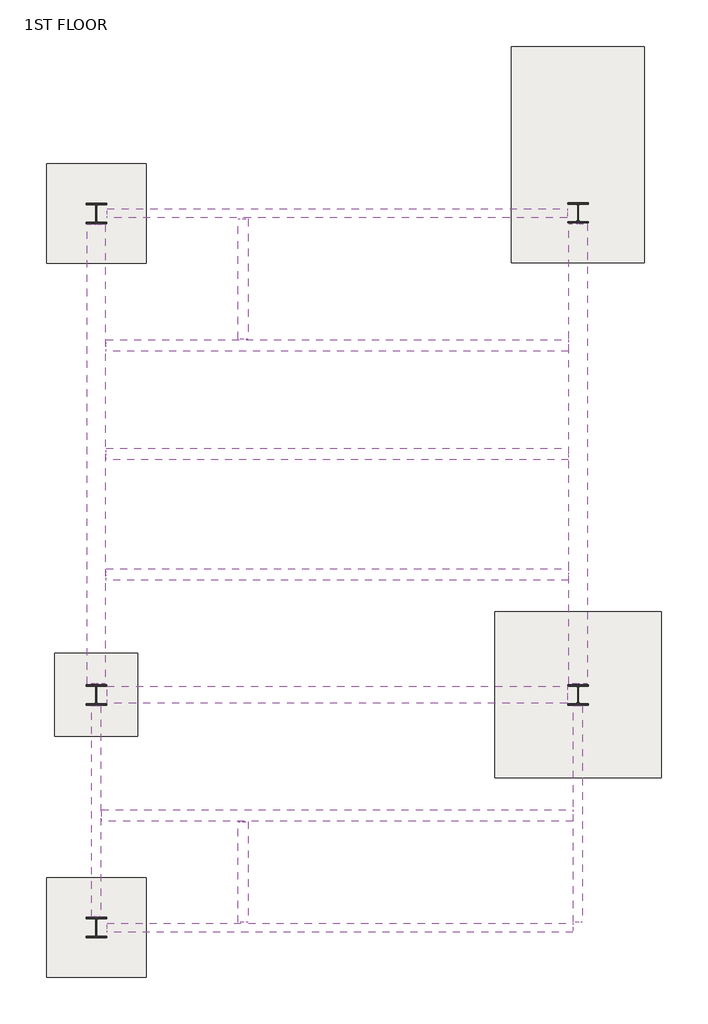
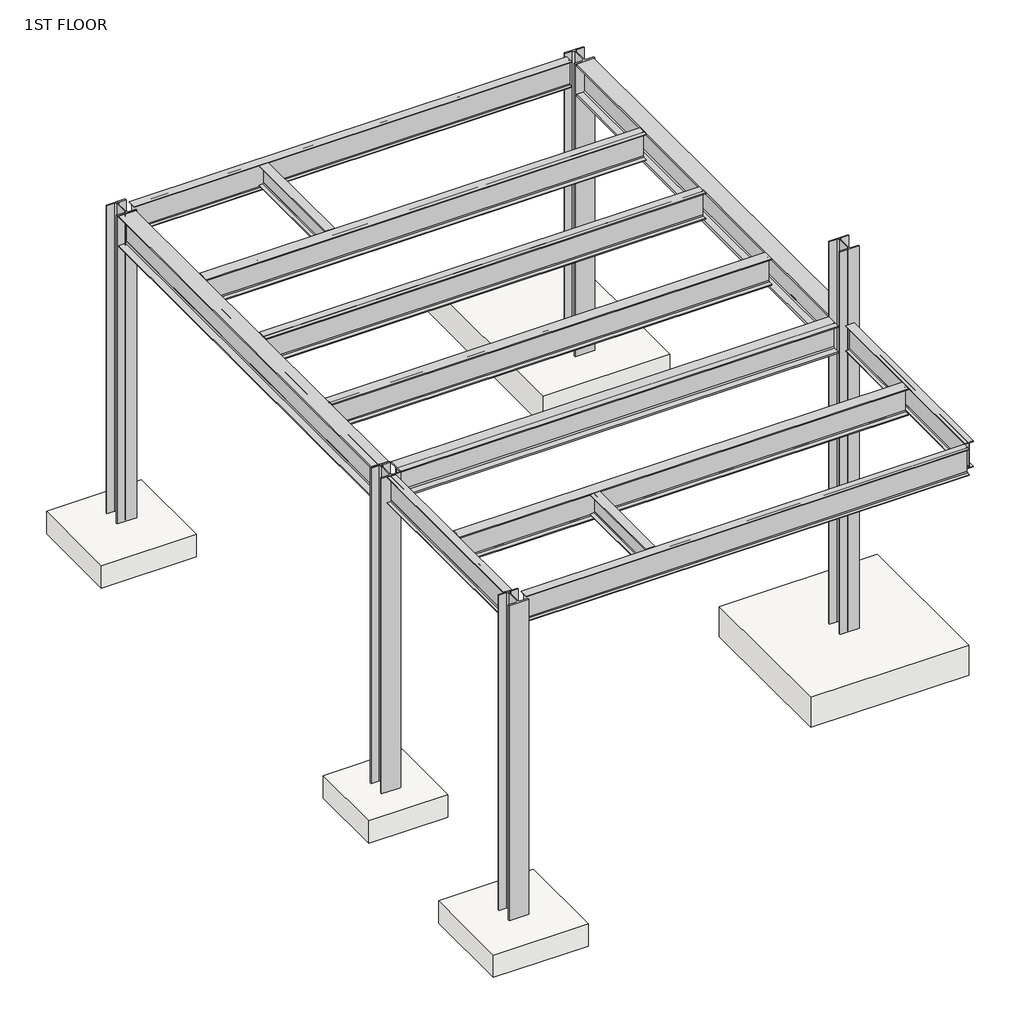
# One storey: 13 beams, 5 columns, 5 slabs.
"""IFC4 building model written with IfcOpenShell, lengths in millimetres."""

import ifcopenshell
import ifcopenshell.guid

model = None  # the IFC model being written
_history = None  # IfcOwnerHistory: only IFC2X3 demands one
_inside = {}  # id of a spatial element -> (the spatial element, [elements in it])
_under = {}  # id of a project, library or spatial element -> (it, [spatial elements below it])
_declared = {}  # id of a project -> (the project, [libraries it declares])
_typed = {}  # id of a type object -> (the type object, [elements of that type])
_made_of = {}  # id of a material, layer set ... -> (it, [elements and type objects made of it])


def new_model(schema):
    """Start an empty IFC model of exactly this schema.

    Asked for "IFC4X3", IfcOpenShell would pick the latest addendum, in which some entities
    have other attributes; the version numbers below select the first issue.
    IFC2X3 requires an IfcOwnerHistory on every rooted entity: one is made here for all.
    """
    global model, _history
    if schema == "IFC4X3":
        model = ifcopenshell.file(schema_version=(4, 3, 0, 0))
    else:
        model = ifcopenshell.file(schema=schema)
    _inside.clear()
    _under.clear()
    _declared.clear()
    _typed.clear()
    _made_of.clear()
    _history = None
    if model.schema == "IFC2X3":
        org = make("IfcOrganization", Name="unknown")
        user = make(
            "IfcPersonAndOrganization",
            ThePerson=make("IfcPerson", FamilyName="unknown"),
            TheOrganization=org,
        )
        app = make(
            "IfcApplication",
            ApplicationDeveloper=org,
            Version="unknown",
            ApplicationFullName="unknown",
            ApplicationIdentifier="unknown",
        )
        _history = make(
            "IfcOwnerHistory",
            OwningUser=user,
            OwningApplication=app,
            ChangeAction="ADDED",
            CreationDate=0,
        )
    return model


def make(cls, **values):
    """One entity of the class cls with the attributes given. An attribute that is None is left unset."""
    return model.create_entity(
        cls, **{name: value for name, value in values.items() if value is not None}
    )


def rooted(cls, **values):
    """An entity with a GlobalId (a new one), such as an element, a storey or a relation."""
    return make(cls, GlobalId=ifcopenshell.guid.new(), OwnerHistory=_history, **values)


def si_unit(unit_type, name, prefix=None):
    """IfcSIUnit, for example si_unit("LENGTHUNIT", "METRE", prefix="MILLI")."""
    return make("IfcSIUnit", UnitType=unit_type, Prefix=prefix, Name=name)


def assignment(units):
    """IfcUnitAssignment: the units of a project."""
    return None if units is None else make("IfcUnitAssignment", Units=units)


def point(xyz):
    """IfcCartesianPoint."""
    return None if xyz is None else make("IfcCartesianPoint", Coordinates=xyz)


def direction(xyz):
    """IfcDirection."""
    return None if xyz is None else make("IfcDirection", DirectionRatios=xyz)


def frame(location, z_axis=None, x_axis=None):
    """IfcAxis2Placement3D, a coordinate frame: its origin and axes. An axis left out is left unset."""
    return make(
        "IfcAxis2Placement3D",
        Location=point(location),
        Axis=direction(z_axis),
        RefDirection=direction(x_axis),
    )


def frame_2d(location, x_axis=None):
    """IfcAxis2Placement2D, a coordinate frame in the plane: its origin and x axis."""
    return make(
        "IfcAxis2Placement2D", Location=point(location), RefDirection=direction(x_axis)
    )


def origin():
    """The frame at (0, 0, 0) with its axes left unset."""
    return frame((0.0, 0.0, 0.0))


def origin_with_axes():
    """The frame at (0, 0, 0) with the z axis (0, 0, 1) and the x axis (1, 0, 0) written out."""
    return frame((0.0, 0.0, 0.0), z_axis=(0.0, 0.0, 1.0), x_axis=(1.0, 0.0, 0.0))


def place(relative_to, where):
    """IfcLocalPlacement: puts the frame where relative to a parent placement (None: the world)."""
    return make(
        "IfcLocalPlacement", PlacementRelTo=relative_to, RelativePlacement=where
    )


def context(
    kind, dimensions, precision=None, world=None, true_north=None, identifier=None
):
    """IfcGeometricRepresentationContext, for example the 3D "Model" context."""
    return make(
        "IfcGeometricRepresentationContext",
        ContextIdentifier=identifier,
        ContextType=kind,
        CoordinateSpaceDimension=dimensions,
        Precision=precision,
        WorldCoordinateSystem=world,
        TrueNorth=true_north,
    )


def project(units=None, contexts=None):
    """IfcProject with its units and contexts."""
    return rooted(
        "IfcProject",
        Name="project",
        RepresentationContexts=contexts,
        UnitsInContext=assignment(units),
    )


def spatial(cls, under=None, at=None, **own):
    """A site, building, storey or space (cls), placed at a placement, below another one or the project."""
    s = rooted(cls, ObjectPlacement=at, **own)
    if under is not None:
        _under.setdefault(under.id(), (under, []))[1].append(s)
    return s


def polyline(points):
    """IfcPolyline through the points."""
    return make("IfcPolyline", Points=[point(p) for p in points])


def circle_curve(where, radius):
    """IfcCircle in the frame where."""
    return make("IfcCircle", Position=where, Radius=radius)


def trimmed(basis, trim1, trim2, sense, master):
    """IfcTrimmedCurve: the piece of a basis curve between two trims."""
    return make(
        "IfcTrimmedCurve",
        BasisCurve=basis,
        Trim1=trim1,
        Trim2=trim2,
        SenseAgreement=sense,
        MasterRepresentation=master,
    )


def segment(curve, same_sense, transition):
    """IfcCompositeCurveSegment."""
    return make(
        "IfcCompositeCurveSegment",
        Transition=transition,
        SameSense=same_sense,
        ParentCurve=curve,
    )


def composite_curve(segments, self_intersect=None):
    """IfcCompositeCurve: segments joined end to end."""
    return make("IfcCompositeCurve", Segments=segments, SelfIntersect=self_intersect)


def outline(outer, holes=None, kind="AREA"):
    """IfcArbitraryClosedProfileDef: a profile drawn as a closed curve; with holes, ...WithVoids."""
    if holes is None:
        return make("IfcArbitraryClosedProfileDef", ProfileType=kind, OuterCurve=outer)
    return make(
        "IfcArbitraryProfileDefWithVoids",
        ProfileType=kind,
        OuterCurve=outer,
        InnerCurves=holes,
    )


def extrude(swept, where, along, depth):
    """IfcExtrudedAreaSolid: the profile swept, set in the frame where, extruded along a direction by depth."""
    return make(
        "IfcExtrudedAreaSolid",
        SweptArea=swept,
        Position=where,
        ExtrudedDirection=direction(along),
        Depth=depth,
    )


def shape(context_of_items, identifier, shape_type, items):
    """IfcShapeRepresentation: the items that make up one representation, for example the "Body"."""
    return make(
        "IfcShapeRepresentation",
        ContextOfItems=context_of_items,
        RepresentationIdentifier=identifier,
        RepresentationType=shape_type,
        Items=items,
    )


def source(mapping_origin, context_of_items, identifier, shape_type, items):
    """IfcRepresentationMap: a shape defined once, which mapped items show again and again."""
    return make(
        "IfcRepresentationMap",
        MappingOrigin=mapping_origin,
        MappedRepresentation=shape(context_of_items, identifier, shape_type, items),
    )


def transform(
    local_origin,
    x_axis=None,
    y_axis=None,
    z_axis=None,
    scale=None,
    scale2=None,
    scale3=None,
    uniform=True,
):
    """IfcCartesianTransformationOperator3D, or its non-uniform kind. x_axis, y_axis, z_axis: its Axis1, 2, 3."""
    if uniform:
        return make(
            "IfcCartesianTransformationOperator3D",
            Axis1=direction(x_axis),
            Axis2=direction(y_axis),
            LocalOrigin=point(local_origin),
            Scale=scale,
            Axis3=direction(z_axis),
        )
    return make(
        "IfcCartesianTransformationOperator3DnonUniform",
        Axis1=direction(x_axis),
        Axis2=direction(y_axis),
        LocalOrigin=point(local_origin),
        Scale=scale,
        Axis3=direction(z_axis),
        Scale2=scale2,
        Scale3=scale3,
    )


def mapped(mapping_source, mapping_target):
    """IfcMappedItem: shows the shape of a source again, moved by a transform."""
    return make(
        "IfcMappedItem", MappingSource=mapping_source, MappingTarget=mapping_target
    )


def made_of(thing, what):
    """Note that an element or type object is made of a material, layer set ...; save() writes the relation."""
    if what is not None:
        _made_of.setdefault(what.id(), (what, []))[1].append(thing)
    return thing


def element(
    cls,
    number,
    at=None,
    inside=None,
    cuts=None,
    type_object=None,
    material=None,
    context=None,
    identifier="Body",
    shape_type=None,
    held_by="IfcProductDefinitionShape",
    body=None,
    shapes=None,
    **own,
):
    """One element of the class cls, such as IfcWall. Its Tag is "e" and its number.

    at: its placement. inside: the storey or other place that contains it. cuts: it is an
    opening in that element (IfcRelVoidsElement). A single representation is given by context,
    identifier, shape_type and body (its items); several are given by shapes. held_by: the class
    of the entity that holds the representations. save() writes the other relations.
    """
    e = rooted(cls, Tag="e%d" % number, ObjectPlacement=at, **own)
    if body is not None:
        shapes = [shape(context, identifier, shape_type, body)]
    if shapes is not None:
        e.Representation = make(held_by, Representations=shapes)
    if inside is not None:
        _inside.setdefault(inside.id(), (inside, []))[1].append(e)
    if cuts is not None:
        rooted(
            "IfcRelVoidsElement", RelatingBuildingElement=cuts, RelatedOpeningElement=e
        )
    if type_object is not None:
        _typed.setdefault(type_object.id(), (type_object, []))[1].append(e)
    return made_of(e, material)


def aggregate(whole, parts):
    """IfcRelAggregates: a whole, such as a stair, and the parts it consists of."""
    return rooted("IfcRelAggregates", RelatingObject=whole, RelatedObjects=parts)


def save(model, path):
    """Write the relations noted so far, then the file.

    IfcRelAggregates (storeys below a building ...), IfcRelContainedInSpatialStructure (elements
    in a storey), IfcRelDefinesByType, IfcRelAssociatesMaterial and IfcRelDeclares: one each for
    every whole, place, type object, material and project.
    """
    for whole, parts in _under.values():
        aggregate(whole, parts)
    for where, things in _inside.values():
        rooted(
            "IfcRelContainedInSpatialStructure",
            RelatedElements=things,
            RelatingStructure=where,
        )
    for kind, things in _typed.values():
        rooted("IfcRelDefinesByType", RelatedObjects=things, RelatingType=kind)
    for what, things in _made_of.values():
        rooted("IfcRelAssociatesMaterial", RelatedObjects=things, RelatingMaterial=what)
    for by, libraries in _declared.values():
        rooted("IfcRelDeclares", RelatingContext=by, RelatedDefinitions=libraries)
    model.write(path)


def w_wide_flange_w16x50_2f8f61bc(model_context):
    return source(origin(), model_context, "Body", "SweptSolid", [
        extrude(outline(composite_curve([segment(polyline([(89.789, -191.008), (89.789, -207.01), (-89.789, -207.01), (-89.789, -191.008), (-22.1615, -191.008)]), True, "CONTINUOUS"), segment(trimmed(circle_curve(frame_2d((-22.1615, -173.6725)), 17.3355), [point((-22.1615, -191.008))], [point((-4.826, -173.6725))], True, "CARTESIAN"), True, "CONTINUOUS"), segment(polyline([(-4.826, -173.6725), (-4.826, 173.6725)]), True, "CONTINUOUS"), segment(trimmed(circle_curve(frame_2d((-22.1615, 173.6725)), 17.3355), [point((-4.826, 173.6725))], [point((-22.1615, 191.008))], True, "CARTESIAN"), True, "CONTINUOUS"), segment(polyline([(-22.1615, 191.008), (-89.789, 191.008), (-89.789, 207.01), (89.789, 207.01), (89.789, 191.008), (22.1615, 191.008)]), True, "CONTINUOUS"), segment(trimmed(circle_curve(frame_2d((22.1615, 173.6725)), 17.3355), [point((22.1615, 191.008))], [point((4.826, 173.6725))], True, "CARTESIAN"), True, "CONTINUOUS"), segment(polyline([(4.826, 173.6725), (4.826, -173.6725)]), True, "CONTINUOUS"), segment(trimmed(circle_curve(frame_2d((22.1615, -173.6725)), 17.3355), [point((4.826, -173.6725))], [point((22.1615, -191.008))], True, "CARTESIAN"), True, "CONTINUOUS"), segment(polyline([(22.1615, -191.008), (89.789, -191.008)]), True, "CONTINUOUS")], self_intersect=False)), frame((-1094.5030758, 0.0, 0.0), z_axis=(1.0, 0.0, 0.0), x_axis=(0.0, 1.0, 0.0)), (0.0, 0.0, 1.0), 2211.8661516),
    ])


def w_wide_flange_w16x50_f430b839(model_context):
    return source(origin(), model_context, "Body", "SweptSolid", [
        extrude(outline(composite_curve([segment(polyline([(-89.789, -191.008), (-22.1615, -191.008)]), True, "CONTINUOUS"), segment(trimmed(circle_curve(frame_2d((-22.1615, -173.6725)), 17.3355), [point((-22.1615, -191.008))], [point((-4.826, -173.6725))], True, "CARTESIAN"), True, "CONTINUOUS"), segment(polyline([(-4.826, -173.6725), (-4.826, 173.6725)]), True, "CONTINUOUS"), segment(trimmed(circle_curve(frame_2d((-22.1615, 173.6725)), 17.3355), [point((-4.826, 173.6725))], [point((-22.1615, 191.008))], True, "CARTESIAN"), True, "CONTINUOUS"), segment(polyline([(-22.1615, 191.008), (-89.789, 191.008), (-89.789, 207.01), (89.789, 207.01), (89.789, 191.008), (22.1615, 191.008)]), True, "CONTINUOUS"), segment(trimmed(circle_curve(frame_2d((22.1615, 173.6725)), 17.3355), [point((22.1615, 191.008))], [point((4.826, 173.6725))], True, "CARTESIAN"), True, "CONTINUOUS"), segment(polyline([(4.826, 173.6725), (4.826, -173.6725)]), True, "CONTINUOUS"), segment(trimmed(circle_curve(frame_2d((22.1615, -173.6725)), 17.3355), [point((4.826, -173.6725))], [point((22.1615, -191.008))], True, "CARTESIAN"), True, "CONTINUOUS"), segment(polyline([(22.1615, -191.008), (89.789, -191.008), (89.789, -207.01), (-89.789, -207.01), (-89.789, -191.008)]), True, "CONTINUOUS")], self_intersect=False)), frame((-912.045346, 0.0, 0.0), z_axis=(1.0, 0.0, 0.0), x_axis=(0.0, 1.0, 0.0)), (0.0, 0.0, 1.0), 1846.950692),
    ])


def w_wide_flange_w21x111_51b1a384(model_context):
    return source(origin(), model_context, "Body", "SweptSolid", [
        extrude(outline(composite_curve([segment(polyline([(156.21, -250.825), (156.21, -273.05), (-156.21, -273.05), (-156.21, -250.825), (-29.21, -250.825)]), True, "CONTINUOUS"), segment(trimmed(circle_curve(frame_2d((-29.21, -228.6)), 22.225), [point((-29.21, -250.825))], [point((-6.985, -228.6))], True, "CARTESIAN"), True, "CONTINUOUS"), segment(polyline([(-6.985, -228.6), (-6.985, 228.6)]), True, "CONTINUOUS"), segment(trimmed(circle_curve(frame_2d((-29.21, 228.6)), 22.225), [point((-6.985, 228.6))], [point((-29.21, 250.825))], True, "CARTESIAN"), True, "CONTINUOUS"), segment(polyline([(-29.21, 250.825), (-156.21, 250.825), (-156.21, 273.05), (156.21, 273.05), (156.21, 250.825), (29.21, 250.825)]), True, "CONTINUOUS"), segment(trimmed(circle_curve(frame_2d((29.21, 228.6)), 22.225), [point((29.21, 250.825))], [point((6.985, 228.6))], True, "CARTESIAN"), True, "CONTINUOUS"), segment(polyline([(6.985, 228.6), (6.985, -228.6)]), True, "CONTINUOUS"), segment(trimmed(circle_curve(frame_2d((29.21, -228.6)), 22.225), [point((6.985, -228.6))], [point((29.21, -250.825))], True, "CARTESIAN"), True, "CONTINUOUS"), segment(polyline([(29.21, -250.825), (156.21, -250.825)]), True, "CONTINUOUS")], self_intersect=False)), frame((-4220.21, 0.0, 0.0), z_axis=(1.0, 0.0, 0.0), x_axis=(0.0, 1.0, 0.0)), (0.0, 0.0, 1.0), 8440.42),
    ])


def w_wide_flange_w21x44_feb090a0(model_context):
    return source(origin(), model_context, "Body", "SweptSolid", [
        extrude(outline(composite_curve([segment(polyline([(82.55, -251.46), (82.55, -262.89), (-82.55, -262.89), (-82.55, -251.46), (-21.59, -251.46)]), True, "CONTINUOUS"), segment(trimmed(circle_curve(frame_2d((-21.59, -234.315)), 17.145), [point((-21.59, -251.46))], [point((-4.445, -234.315))], True, "CARTESIAN"), True, "CONTINUOUS"), segment(polyline([(-4.445, -234.315), (-4.445, 234.315)]), True, "CONTINUOUS"), segment(trimmed(circle_curve(frame_2d((-21.59, 234.315)), 17.145), [point((-4.445, 234.315))], [point((-21.59, 251.46))], True, "CARTESIAN"), True, "CONTINUOUS"), segment(polyline([(-21.59, 251.46), (-82.55, 251.46), (-82.55, 262.89), (82.55, 262.89), (82.55, 251.46), (21.59, 251.46)]), True, "CONTINUOUS"), segment(trimmed(circle_curve(frame_2d((21.59, 234.315)), 17.145), [point((21.59, 251.46))], [point((4.445, 234.315))], True, "CARTESIAN"), True, "CONTINUOUS"), segment(polyline([(4.445, 234.315), (4.445, -234.315)]), True, "CONTINUOUS"), segment(trimmed(circle_curve(frame_2d((21.59, -234.315)), 17.145), [point((4.445, -234.315))], [point((21.59, -251.46))], True, "CARTESIAN"), True, "CONTINUOUS"), segment(polyline([(21.59, -251.46), (82.55, -251.46)]), True, "CONTINUOUS")], self_intersect=False)), frame((-4220.21, 0.0, 0.0), z_axis=(1.0, 0.0, 0.0), x_axis=(0.0, 1.0, 0.0)), (0.0, 0.0, 1.0), 8440.42),
    ])


def w_wide_flange_w21x44_b9bda158(model_context):
    return source(origin(), model_context, "Body", "SweptSolid", [
        extrude(outline(composite_curve([segment(polyline([(82.55, -251.46), (82.55, -262.89), (-82.55, -262.89), (-82.55, -251.46), (-21.59, -251.46)]), True, "CONTINUOUS"), segment(trimmed(circle_curve(frame_2d((-21.59, -234.315)), 17.145), [point((-21.59, -251.46))], [point((-4.445, -234.315))], True, "CARTESIAN"), True, "CONTINUOUS"), segment(polyline([(-4.445, -234.315), (-4.445, 234.315)]), True, "CONTINUOUS"), segment(trimmed(circle_curve(frame_2d((-21.59, 234.315)), 17.145), [point((-4.445, 234.315))], [point((-21.59, 251.46))], True, "CARTESIAN"), True, "CONTINUOUS"), segment(polyline([(-21.59, 251.46), (-82.55, 251.46), (-82.55, 262.89), (82.55, 262.89), (82.55, 251.46), (21.59, 251.46)]), True, "CONTINUOUS"), segment(trimmed(circle_curve(frame_2d((21.59, 234.315)), 17.145), [point((21.59, 251.46))], [point((4.445, 234.315))], True, "CARTESIAN"), True, "CONTINUOUS"), segment(polyline([(4.445, 234.315), (4.445, -234.315)]), True, "CONTINUOUS"), segment(trimmed(circle_curve(frame_2d((21.59, -234.315)), 17.145), [point((4.445, -234.315))], [point((21.59, -251.46))], True, "CARTESIAN"), True, "CONTINUOUS"), segment(polyline([(21.59, -251.46), (82.55, -251.46)]), True, "CONTINUOUS")], self_intersect=False)), frame((-1935.665346, 0.0, 0.0), z_axis=(1.0, 0.0, 0.0), x_axis=(0.0, 1.0, 0.0)), (0.0, 0.0, 1.0), 3868.155692),
    ])


def w_wide_flange_w21x44_85607f17(model_context):
    return source(origin(), model_context, "Body", "SweptSolid", [
        extrude(outline(composite_curve([segment(polyline([(82.55, -251.46), (82.55, -262.89), (-82.55, -262.89), (-82.55, -251.46), (-21.59, -251.46)]), True, "CONTINUOUS"), segment(trimmed(circle_curve(frame_2d((-21.59, -234.315)), 17.145), [point((-21.59, -251.46))], [point((-4.445, -234.315))], True, "CARTESIAN"), True, "CONTINUOUS"), segment(polyline([(-4.445, -234.315), (-4.445, 234.315)]), True, "CONTINUOUS"), segment(trimmed(circle_curve(frame_2d((-21.59, 234.315)), 17.145), [point((-4.445, 234.315))], [point((-21.59, 251.46))], True, "CARTESIAN"), True, "CONTINUOUS"), segment(polyline([(-21.59, 251.46), (-82.55, 251.46), (-82.55, 262.89), (82.55, 262.89), (82.55, 251.46), (21.59, 251.46)]), True, "CONTINUOUS"), segment(trimmed(circle_curve(frame_2d((21.59, 234.315)), 17.145), [point((21.59, 251.46))], [point((4.445, 234.315))], True, "CARTESIAN"), True, "CONTINUOUS"), segment(polyline([(4.445, 234.315), (4.445, -234.315)]), True, "CONTINUOUS"), segment(trimmed(circle_curve(frame_2d((21.59, -234.315)), 17.145), [point((4.445, -234.315))], [point((21.59, -251.46))], True, "CARTESIAN"), True, "CONTINUOUS"), segment(polyline([(21.59, -251.46), (82.55, -251.46)]), True, "CONTINUOUS")], self_intersect=False)), frame((-2039.805346, 0.0, 0.0), z_axis=(1.0, 0.0, 0.0), x_axis=(0.0, 1.0, 0.0)), (0.0, 0.0, 1.0), 3975.470692),
    ])


def w_wide_flange_w21x44_87bcda2b(model_context):
    return source(origin(), model_context, "Body", "SweptSolid", [
        extrude(outline(composite_curve([segment(polyline([(82.55, -251.46), (82.55, -262.89), (-82.55, -262.89), (-82.55, -251.46), (-21.59, -251.46)]), True, "CONTINUOUS"), segment(trimmed(circle_curve(frame_2d((-21.59, -234.315)), 17.145), [point((-21.59, -251.46))], [point((-4.445, -234.315))], True, "CARTESIAN"), True, "CONTINUOUS"), segment(polyline([(-4.445, -234.315), (-4.445, 234.315)]), True, "CONTINUOUS"), segment(trimmed(circle_curve(frame_2d((-21.59, 234.315)), 17.145), [point((-4.445, 234.315))], [point((-21.59, 251.46))], True, "CARTESIAN"), True, "CONTINUOUS"), segment(polyline([(-21.59, 251.46), (-82.55, 251.46), (-82.55, 262.89), (82.55, 262.89), (82.55, 251.46), (21.59, 251.46)]), True, "CONTINUOUS"), segment(trimmed(circle_curve(frame_2d((21.59, 234.315)), 17.145), [point((21.59, 251.46))], [point((4.445, 234.315))], True, "CARTESIAN"), True, "CONTINUOUS"), segment(polyline([(4.445, 234.315), (4.445, -234.315)]), True, "CONTINUOUS"), segment(trimmed(circle_curve(frame_2d((21.59, -234.315)), 17.145), [point((4.445, -234.315))], [point((21.59, -251.46))], True, "CARTESIAN"), True, "CONTINUOUS"), segment(polyline([(21.59, -251.46), (82.55, -251.46)]), True, "CONTINUOUS")], self_intersect=False)), frame((-4220.21, 0.0, 0.0), z_axis=(1.0, 0.0, 0.0), x_axis=(0.0, 1.0, 0.0)), (0.0, 0.0, 1.0), 8544.56),
    ])


def w_wide_flange_w21x73_23efea6e(model_context):
    return source(origin(), model_context, "Body", "SweptSolid", [
        extrude(outline(composite_curve([segment(polyline([(105.41, -250.444), (105.41, -269.24), (-105.41, -269.24), (-105.41, -250.444), (-23.495, -250.444)]), True, "CONTINUOUS"), segment(trimmed(circle_curve(frame_2d((-23.495, -232.7275)), 17.7165), [point((-23.495, -250.444))], [point((-5.7785, -232.7275))], True, "CARTESIAN"), True, "CONTINUOUS"), segment(polyline([(-5.7785, -232.7275), (-5.7785, 232.7275)]), True, "CONTINUOUS"), segment(trimmed(circle_curve(frame_2d((-23.495, 232.7275)), 17.7165), [point((-5.7785, 232.7275))], [point((-23.495, 250.444))], True, "CARTESIAN"), True, "CONTINUOUS"), segment(polyline([(-23.495, 250.444), (-105.41, 250.444), (-105.41, 269.24), (105.41, 269.24), (105.41, 250.444), (23.495, 250.444)]), True, "CONTINUOUS"), segment(trimmed(circle_curve(frame_2d((23.495, 232.7275)), 17.7165), [point((23.495, 250.444))], [point((5.7785, 232.7275))], True, "CARTESIAN"), True, "CONTINUOUS"), segment(polyline([(5.7785, 232.7275), (5.7785, -232.7275)]), True, "CONTINUOUS"), segment(trimmed(circle_curve(frame_2d((23.495, -232.7275)), 17.7165), [point((5.7785, -232.7275))], [point((23.495, -250.444))], True, "CARTESIAN"), True, "CONTINUOUS"), segment(polyline([(23.495, -250.444), (105.41, -250.444)]), True, "CONTINUOUS")], self_intersect=False)), frame((-4324.35, 0.0, 0.0), z_axis=(1.0, 0.0, 0.0), x_axis=(0.0, 1.0, 0.0)), (0.0, 0.0, 1.0), 8648.7),
    ])


def w_wide_flange_w21x73_6fdf119d(model_context):
    return source(origin(), model_context, "Body", "SweptSolid", [
        extrude(outline(composite_curve([segment(polyline([(105.41, -250.444), (105.41, -269.24), (-105.41, -269.24), (-105.41, -250.444), (-23.495, -250.444)]), True, "CONTINUOUS"), segment(trimmed(circle_curve(frame_2d((-23.495, -232.7275)), 17.7165), [point((-23.495, -250.444))], [point((-5.7785, -232.7275))], True, "CARTESIAN"), True, "CONTINUOUS"), segment(polyline([(-5.7785, -232.7275), (-5.7785, 232.7275)]), True, "CONTINUOUS"), segment(trimmed(circle_curve(frame_2d((-23.495, 232.7275)), 17.7165), [point((-5.7785, 232.7275))], [point((-23.495, 250.444))], True, "CARTESIAN"), True, "CONTINUOUS"), segment(polyline([(-23.495, 250.444), (-105.41, 250.444), (-105.41, 269.24), (105.41, 269.24), (105.41, 250.444), (23.495, 250.444)]), True, "CONTINUOUS"), segment(trimmed(circle_curve(frame_2d((23.495, 232.7275)), 17.7165), [point((23.495, 250.444))], [point((5.7785, 232.7275))], True, "CARTESIAN"), True, "CONTINUOUS"), segment(polyline([(5.7785, 232.7275), (5.7785, -232.7275)]), True, "CONTINUOUS"), segment(trimmed(circle_curve(frame_2d((23.495, -232.7275)), 17.7165), [point((5.7785, -232.7275))], [point((23.495, -250.444))], True, "CARTESIAN"), True, "CONTINUOUS"), segment(polyline([(23.495, -250.444), (105.41, -250.444)]), True, "CONTINUOUS")], self_intersect=False)), frame((-4243.07, 0.0, 0.0), z_axis=(1.0, 0.0, 0.0), x_axis=(0.0, 1.0, 0.0)), (0.0, 0.0, 1.0), 8483.6),
    ])


def w_wide_flange_w24x131_18549e9f(model_context):
    return source(origin(), model_context, "Body", "SweptSolid", [
        extrude(outline(composite_curve([segment(polyline([(163.83, -286.766), (163.83, -311.15), (-163.83, -311.15), (-163.83, -286.766), (-30.9245, -286.766)]), True, "CONTINUOUS"), segment(trimmed(circle_curve(frame_2d((-30.9245, -263.525)), 23.241), [point((-30.9245, -286.766))], [point((-7.6835, -263.525))], True, "CARTESIAN"), True, "CONTINUOUS"), segment(polyline([(-7.6835, -263.525), (-7.6835, 263.525)]), True, "CONTINUOUS"), segment(trimmed(circle_curve(frame_2d((-30.9245, 263.525)), 23.241), [point((-7.6835, 263.525))], [point((-30.9245, 286.766))], True, "CARTESIAN"), True, "CONTINUOUS"), segment(polyline([(-30.9245, 286.766), (-163.83, 286.766), (-163.83, 311.15), (163.83, 311.15), (163.83, 286.766), (30.9245, 286.766)]), True, "CONTINUOUS"), segment(trimmed(circle_curve(frame_2d((30.9245, 263.525)), 23.241), [point((30.9245, 286.766))], [point((7.6835, 263.525))], True, "CARTESIAN"), True, "CONTINUOUS"), segment(polyline([(7.6835, 263.525), (7.6835, -263.525)]), True, "CONTINUOUS"), segment(trimmed(circle_curve(frame_2d((30.9245, -263.525)), 23.241), [point((7.6835, -263.525))], [point((30.9245, -286.766))], True, "CARTESIAN"), True, "CONTINUOUS"), segment(polyline([(30.9245, -286.766), (163.83, -286.766)]), True, "CONTINUOUS")], self_intersect=False)), frame((-4213.6230758, 0.0, 0.0), z_axis=(1.0, 0.0, 0.0), x_axis=(0.0, 1.0, 0.0)), (0.0, 0.0, 1.0), 8427.2461516),
    ])


def w_wide_flange_w24x229_264a0a21(model_context):
    return source(origin(), model_context, "Body", "SweptSolid", [
        extrude(outline(composite_curve([segment(polyline([(166.37, -286.258), (166.37, -330.2), (-166.37, -330.2), (-166.37, -286.258), (-34.925, -286.258)]), True, "CONTINUOUS"), segment(trimmed(circle_curve(frame_2d((-34.925, -263.525)), 22.733), [point((-34.925, -286.258))], [point((-12.192, -263.525))], True, "CARTESIAN"), True, "CONTINUOUS"), segment(polyline([(-12.192, -263.525), (-12.192, 263.525)]), True, "CONTINUOUS"), segment(trimmed(circle_curve(frame_2d((-34.925, 263.525)), 22.733), [point((-12.192, 263.525))], [point((-34.925, 286.258))], True, "CARTESIAN"), True, "CONTINUOUS"), segment(polyline([(-34.925, 286.258), (-166.37, 286.258), (-166.37, 330.2), (166.37, 330.2), (166.37, 286.258), (34.925, 286.258)]), True, "CONTINUOUS"), segment(trimmed(circle_curve(frame_2d((34.925, 263.525)), 22.733), [point((34.925, 286.258))], [point((12.192, 263.525))], True, "CARTESIAN"), True, "CONTINUOUS"), segment(polyline([(12.192, 263.525), (12.192, -263.525)]), True, "CONTINUOUS"), segment(trimmed(circle_curve(frame_2d((34.925, -263.525)), 22.733), [point((12.192, -263.525))], [point((34.925, -286.258))], True, "CARTESIAN"), True, "CONTINUOUS"), segment(polyline([(34.925, -286.258), (166.37, -286.258)]), True, "CONTINUOUS")], self_intersect=False)), frame((-4220.21, 0.0, 0.0), z_axis=(1.0, 0.0, 0.0), x_axis=(0.0, 1.0, 0.0)), (0.0, 0.0, 1.0), 8440.42),
    ])


def w_wide_flange_column_w14x132_97c2514c(model_context):
    return source(origin(), model_context, "Body", "SweptSolid", [
        extrude(outline(composite_curve([segment(polyline([(186.69, 186.69), (186.69, 160.528), (40.767, 160.528)]), True, "CONTINUOUS"), segment(trimmed(circle_curve(frame_2d((40.767, 127.9525)), 32.5755), [point((40.767, 160.528))], [point((8.1915, 127.9525))], True, "CARTESIAN"), True, "CONTINUOUS"), segment(polyline([(8.1915, 127.9525), (8.1915, -127.9525)]), True, "CONTINUOUS"), segment(trimmed(circle_curve(frame_2d((40.767, -127.9525)), 32.5755), [point((8.1915, -127.9525))], [point((40.767, -160.528))], True, "CARTESIAN"), True, "CONTINUOUS"), segment(polyline([(40.767, -160.528), (186.69, -160.528), (186.69, -186.69), (-186.69, -186.69), (-186.69, -160.528), (-40.767, -160.528)]), True, "CONTINUOUS"), segment(trimmed(circle_curve(frame_2d((-40.767, -127.9525)), 32.5755), [point((-40.767, -160.528))], [point((-8.1915, -127.9525))], True, "CARTESIAN"), True, "CONTINUOUS"), segment(polyline([(-8.1915, -127.9525), (-8.1915, 127.9525)]), True, "CONTINUOUS"), segment(trimmed(circle_curve(frame_2d((-40.767, 127.9525)), 32.5755), [point((-8.1915, 127.9525))], [point((-40.767, 160.528))], True, "CARTESIAN"), True, "CONTINUOUS"), segment(polyline([(-40.767, 160.528), (-186.69, 160.528), (-186.69, 186.69), (186.69, 186.69)]), True, "CONTINUOUS")], self_intersect=False)), frame((0.0, 0.0, -304.8), z_axis=(0.0, 0.0, 1.0), x_axis=(1.0, 0.0, 0.0)), (0.0, 0.0, 1.0), 7797.8),
    ])


def w_wide_flange_column_w14x132_1d26bb89(model_context):
    return source(origin(), model_context, "Body", "SweptSolid", [
        extrude(outline(composite_curve([segment(polyline([(186.69, -186.69), (-186.69, -186.69), (-186.69, -160.528), (-40.767, -160.528)]), True, "CONTINUOUS"), segment(trimmed(circle_curve(frame_2d((-40.767, -127.9525)), 32.5755), [point((-40.767, -160.528))], [point((-8.1915, -127.9525))], True, "CARTESIAN"), True, "CONTINUOUS"), segment(polyline([(-8.1915, -127.9525), (-8.1915, 127.9525)]), True, "CONTINUOUS"), segment(trimmed(circle_curve(frame_2d((-40.767, 127.9525)), 32.5755), [point((-8.1915, 127.9525))], [point((-40.767, 160.528))], True, "CARTESIAN"), True, "CONTINUOUS"), segment(polyline([(-40.767, 160.528), (-186.69, 160.528), (-186.69, 186.69), (186.69, 186.69), (186.69, 160.528), (40.767, 160.528)]), True, "CONTINUOUS"), segment(trimmed(circle_curve(frame_2d((40.767, 127.9525)), 32.5755), [point((40.767, 160.528))], [point((8.1915, 127.9525))], True, "CARTESIAN"), True, "CONTINUOUS"), segment(polyline([(8.1915, 127.9525), (8.1915, -127.9525)]), True, "CONTINUOUS"), segment(trimmed(circle_curve(frame_2d((40.767, -127.9525)), 32.5755), [point((8.1915, -127.9525))], [point((40.767, -160.528))], True, "CARTESIAN"), True, "CONTINUOUS"), segment(polyline([(40.767, -160.528), (186.69, -160.528), (186.69, -186.69)]), True, "CONTINUOUS")], self_intersect=False)), frame((0.0, 0.0, -304.8), z_axis=(0.0, 0.0, 1.0), x_axis=(1.0, 0.0, 0.0)), (0.0, 0.0, 1.0), 6273.8),
    ])


def w_wide_flange_column_w14x132_b8660559(model_context):
    return source(origin(), model_context, "Body", "SweptSolid", [
        extrude(outline(composite_curve([segment(polyline([(186.69, -186.69), (-186.69, -186.69), (-186.69, -160.528), (-40.767, -160.528)]), True, "CONTINUOUS"), segment(trimmed(circle_curve(frame_2d((-40.767, -127.9525)), 32.5755), [point((-40.767, -160.528))], [point((-8.1915, -127.9525))], True, "CARTESIAN"), True, "CONTINUOUS"), segment(polyline([(-8.1915, -127.9525), (-8.1915, 127.9525)]), True, "CONTINUOUS"), segment(trimmed(circle_curve(frame_2d((-40.767, 127.9525)), 32.5755), [point((-8.1915, 127.9525))], [point((-40.767, 160.528))], True, "CARTESIAN"), True, "CONTINUOUS"), segment(polyline([(-40.767, 160.528), (-186.69, 160.528), (-186.69, 186.69), (186.69, 186.69), (186.69, 160.528), (40.767, 160.528)]), True, "CONTINUOUS"), segment(trimmed(circle_curve(frame_2d((40.767, 127.9525)), 32.5755), [point((40.767, 160.528))], [point((8.1915, 127.9525))], True, "CARTESIAN"), True, "CONTINUOUS"), segment(polyline([(8.1915, 127.9525), (8.1915, -127.9525)]), True, "CONTINUOUS"), segment(trimmed(circle_curve(frame_2d((40.767, -127.9525)), 32.5755), [point((8.1915, -127.9525))], [point((40.767, -160.528))], True, "CARTESIAN"), True, "CONTINUOUS"), segment(polyline([(40.767, -160.528), (186.69, -160.528), (186.69, -186.69)]), True, "CONTINUOUS")], self_intersect=False)), frame((0.0, 0.0, -457.2), z_axis=(0.0, 0.0, 1.0), x_axis=(1.0, 0.0, 0.0)), (0.0, 0.0, 1.0), 6426.2),
    ])


def w_wide_flange_column_w14x132_17457bbd(model_context):
    return source(origin(), model_context, "Body", "SweptSolid", [
        extrude(outline(composite_curve([segment(polyline([(186.69, 186.69), (186.69, 160.528), (40.767, 160.528)]), True, "CONTINUOUS"), segment(trimmed(circle_curve(frame_2d((40.767, 127.9525)), 32.5755), [point((40.767, 160.528))], [point((8.1915, 127.9525))], True, "CARTESIAN"), True, "CONTINUOUS"), segment(polyline([(8.1915, 127.9525), (8.1915, -127.9525)]), True, "CONTINUOUS"), segment(trimmed(circle_curve(frame_2d((40.767, -127.9525)), 32.5755), [point((8.1915, -127.9525))], [point((40.767, -160.528))], True, "CARTESIAN"), True, "CONTINUOUS"), segment(polyline([(40.767, -160.528), (186.69, -160.528), (186.69, -186.69), (-186.69, -186.69), (-186.69, -160.528), (-40.767, -160.528)]), True, "CONTINUOUS"), segment(trimmed(circle_curve(frame_2d((-40.767, -127.9525)), 32.5755), [point((-40.767, -160.528))], [point((-8.1915, -127.9525))], True, "CARTESIAN"), True, "CONTINUOUS"), segment(polyline([(-8.1915, -127.9525), (-8.1915, 127.9525)]), True, "CONTINUOUS"), segment(trimmed(circle_curve(frame_2d((-40.767, 127.9525)), 32.5755), [point((-8.1915, 127.9525))], [point((-40.767, 160.528))], True, "CARTESIAN"), True, "CONTINUOUS"), segment(polyline([(-40.767, 160.528), (-186.69, 160.528), (-186.69, 186.69), (186.69, 186.69)]), True, "CONTINUOUS")], self_intersect=False)), origin_with_axes(), (0.0, 0.0, 1.0), 5969.0),
    ])


def footing_rectangular_1b3ddeb7(model_context):
    return source(origin(), model_context, "Body", "SweptSolid", [
        extrude(outline(polyline([(1219.2, -1981.2), (-1219.2, -1981.2), (-1219.2, 1981.2), (1219.2, 1981.2), (1219.2, -1981.2)])), frame((0.0, 0.0, -609.6), z_axis=(0.0, 0.0, 1.0), x_axis=(1.0, 0.0, 0.0)), (0.0, 0.0, 1.0), 609.6),
    ])


def slab_5ce8dbd1(model_context):
    return source(origin(), model_context, "Body", "SweptSolid", [
        extrude(outline(polyline([(1524.0, 1524.0), (1524.0, -1524.0), (-1524.0, -1524.0), (-1524.0, 1524.0), (1524.0, 1524.0)])), frame((0.0, 0.0, -609.6), z_axis=(0.0, 0.0, 1.0), x_axis=(1.0, 0.0, 0.0)), (0.0, 0.0, 1.0), 609.6),
    ])


model = new_model("IFC4")

# Units and contexts
model_context = context("Model", 3, world=origin())
ifc_project = project(units=[si_unit("LENGTHUNIT", "METRE", prefix="MILLI")], contexts=[model_context])

# Site, building, storey
site = spatial("IfcSite", under=ifc_project)
building = spatial("IfcBuilding", under=site)
storey = spatial("IfcBuildingStorey", under=building, Name="1ST FLOOR", Elevation=0.0)

# Beams
placement = place(None, origin())
w_wide_flange_w16x50_shape = w_wide_flange_w16x50_2f8f61bc(model_context)
element("IfcBeam", 1, ObjectType="W-Wide Flange : W16X50", at=placement, inside=storey, context=model_context, shape_type="MappedRepresentation", body=[
    mapped(w_wide_flange_w16x50_shape, transform((2997.2, 53333.4130758, 5761.99), x_axis=(0.0, 1.0, 0.0), y_axis=(-1.0, 0.0, 0.0), z_axis=(0.0, 0.0, 1.0))),
])
w_wide_flange_w16x50_2_shape = w_wide_flange_w16x50_f430b839(model_context)
element("IfcBeam", 2, ObjectType="W-Wide Flange : W16X50", at=placement, inside=storey, context=model_context, shape_type="MappedRepresentation", body=[
    mapped(w_wide_flange_w16x50_2_shape, transform((2997.2, 42480.044654, 5761.99), x_axis=(0.0, -1.0, 0.0), y_axis=(1.0, 0.0, 0.0), z_axis=(0.0, 0.0, 1.0))),
])
w_wide_flange_w21x111_shape = w_wide_flange_w21x111_51b1a384(model_context)
element("IfcBeam", 3, ObjectType="W-Wide Flange : W21X111", at=placement, inside=storey, context=model_context, shape_type="MappedRepresentation", body=[
    mapped(w_wide_flange_w21x111_shape, transform((4724.4, 45720.0, 5695.95), x_axis=(-1.0, 0.0, 0.0), y_axis=(0.0, -1.0, 0.0), z_axis=(0.0, 0.0, 1.0))),
])
w_wide_flange_w21x44_shape = w_wide_flange_w21x44_feb090a0(model_context)
element("IfcBeam", 4, ObjectType="W-Wide Flange : W21X44", at=placement, inside=storey, context=model_context, shape_type="MappedRepresentation", body=[
    mapped(w_wide_flange_w21x44_shape, transform((4724.4, 54546.0261516, 5706.11), x_axis=(1.0, 0.0, 0.0), y_axis=(0.0, 1.0, 0.0), z_axis=(0.0, 0.0, 1.0))),
])
w_wide_flange_w21x44_2_shape = w_wide_flange_w21x44_b9bda158(model_context)
element("IfcBeam", 5, ObjectType="W-Wide Flange : W21X44", at=placement, inside=storey, context=model_context, shape_type="MappedRepresentation", body=[
    mapped(w_wide_flange_w21x44_2_shape, transform((304.8, 43584.944654, 5706.11), x_axis=(0.0, -1.0, 0.0), y_axis=(1.0, 0.0, 0.0), z_axis=(0.0, 0.0, 1.0))),
])
w_wide_flange_w21x44_3_shape = w_wide_flange_w21x44_85607f17(model_context)
element("IfcBeam", 6, ObjectType="W-Wide Flange : W21X44", at=placement, inside=storey, context=model_context, shape_type="MappedRepresentation", body=[
    mapped(w_wide_flange_w21x44_3_shape, transform((9144.0, 43584.944654, 5706.11), x_axis=(0.0, 1.0, 0.0), y_axis=(-1.0, 0.0, 0.0), z_axis=(0.0, 0.0, 1.0))),
])
w_wide_flange_w21x44_4_shape = w_wide_flange_w21x44_87bcda2b(model_context)
element("IfcBeam", 7, ObjectType="W-Wide Flange : W21X44", at=placement, inside=storey, context=model_context, shape_type="MappedRepresentation", body=[
    mapped(w_wide_flange_w21x44_4_shape, transform((4724.4, 41449.889308, 5706.11), x_axis=(1.0, 0.0, 0.0), y_axis=(0.0, 1.0, 0.0), z_axis=(0.0, 0.0, 1.0))),
])
w_wide_flange_w21x73_shape = w_wide_flange_w21x73_23efea6e(model_context)
element("IfcBeam", 8, ObjectType="W-Wide Flange : W21X73", at=placement, inside=storey, context=model_context, shape_type="MappedRepresentation", body=[
    mapped(w_wide_flange_w21x73_shape, transform((4724.4, 43510.2, 5699.76), x_axis=(-1.0, 0.0, 0.0), y_axis=(0.0, -1.0, 0.0), z_axis=(0.0, 0.0, 1.0))),
])
w_wide_flange_w21x73_2_shape = w_wide_flange_w21x73_6fdf119d(model_context)
element("IfcBeam", 9, ObjectType="W-Wide Flange : W21X73", at=placement, inside=storey, context=model_context, shape_type="MappedRepresentation", body=[
    mapped(w_wide_flange_w21x73_2_shape, transform((4724.4, 52120.8, 5699.76), x_axis=(1.0, 0.0, 0.0), y_axis=(0.0, 1.0, 0.0), z_axis=(0.0, 0.0, 1.0))),
])
element("IfcBeam", 10, ObjectType="W-Wide Flange : W21X73", at=placement, inside=storey, context=model_context, shape_type="MappedRepresentation", body=[
    mapped(w_wide_flange_w21x73_2_shape, transform((4724.4, 50139.6, 5699.76), x_axis=(1.0, 0.0, 0.0), y_axis=(0.0, 1.0, 0.0), z_axis=(0.0, 0.0, 1.0))),
])
element("IfcBeam", 11, ObjectType="W-Wide Flange : W21X73", at=placement, inside=storey, context=model_context, shape_type="MappedRepresentation", body=[
    mapped(w_wide_flange_w21x73_2_shape, transform((4724.4, 47929.8, 5699.76), x_axis=(1.0, 0.0, 0.0), y_axis=(0.0, 1.0, 0.0), z_axis=(0.0, 0.0, 1.0))),
])
w_wide_flange_w24x131_shape = w_wide_flange_w24x131_18549e9f(model_context)
element("IfcBeam", 12, ObjectType="W-Wide Flange : W24X131", at=placement, inside=storey, context=model_context, shape_type="MappedRepresentation", body=[
    mapped(w_wide_flange_w24x131_shape, transform((304.8, 50133.0130758, 5657.85), x_axis=(0.0, -1.0, 0.0), y_axis=(1.0, 0.0, 0.0), z_axis=(0.0, 0.0, 1.0))),
])
w_wide_flange_w24x229_shape = w_wide_flange_w24x229_264a0a21(model_context)
element("IfcBeam", 13, ObjectType="W-Wide Flange : W24X229", at=placement, inside=storey, context=model_context, shape_type="MappedRepresentation", body=[
    mapped(w_wide_flange_w24x229_shape, transform((9144.0, 50139.6, 5638.8), x_axis=(0.0, 1.0, 0.0), y_axis=(-1.0, 0.0, 0.0), z_axis=(0.0, 0.0, 1.0))),
])

# Columns
w_wide_flange_column_w14x132_shape = w_wide_flange_column_w14x132_97c2514c(model_context)
element("IfcColumn", 14, ObjectType="W-Wide Flange-Column : W14X132", at=placement, inside=storey, context=model_context, shape_type="MappedRepresentation", body=[
    mapped(w_wide_flange_column_w14x132_shape, transform((9144.0, 45720.0, 0.0), x_axis=(1.0, 0.0, 0.0), y_axis=(0.0, 1.0, 0.0), z_axis=(0.0, 0.0, 1.0))),
])
w_wide_flange_column_w14x132_2_shape = w_wide_flange_column_w14x132_1d26bb89(model_context)
element("IfcColumn", 15, ObjectType="W-Wide Flange-Column : W14X132", at=placement, inside=storey, context=model_context, shape_type="MappedRepresentation", body=[
    mapped(w_wide_flange_column_w14x132_2_shape, transform((304.8, 54546.0261516, 0.0), x_axis=(1.0, 0.0, 0.0), y_axis=(0.0, 1.0, 0.0), z_axis=(0.0, 0.0, 1.0))),
])
w_wide_flange_column_w14x132_3_shape = w_wide_flange_column_w14x132_b8660559(model_context)
element("IfcColumn", 16, ObjectType="W-Wide Flange-Column : W14X132", at=placement, inside=storey, context=model_context, shape_type="MappedRepresentation", body=[
    mapped(w_wide_flange_column_w14x132_3_shape, transform((304.8, 41453.064308, 0.0), x_axis=(1.0, 0.0, 0.0), y_axis=(0.0, 1.0, 0.0), z_axis=(0.0, 0.0, 1.0))),
])
element("IfcColumn", 17, ObjectType="W-Wide Flange-Column : W14X132", at=placement, inside=storey, context=model_context, shape_type="MappedRepresentation", body=[
    mapped(w_wide_flange_column_w14x132_3_shape, transform((304.8, 45720.0, 0.0), x_axis=(1.0, 0.0, 0.0), y_axis=(0.0, 1.0, 0.0), z_axis=(0.0, 0.0, 1.0))),
])
w_wide_flange_column_w14x132_4_shape = w_wide_flange_column_w14x132_17457bbd(model_context)
element("IfcColumn", 18, ObjectType="W-Wide Flange-Column : W14X132", at=placement, inside=storey, context=model_context, shape_type="MappedRepresentation", body=[
    mapped(w_wide_flange_column_w14x132_4_shape, transform((9144.0, 54559.2, 0.0), x_axis=(1.0, 0.0, 0.0), y_axis=(0.0, 1.0, 0.0), z_axis=(0.0, 0.0, 1.0))),
])

# Slabs
element("IfcSlab", 19, ObjectType="Footing-Rectangular : 6'-0\" x 6''-0\"", at=placement, inside=storey, context=model_context, shape_type="SweptSolid", body=[
    extrude(outline(polyline([(-609.6000003, 53631.6261513), (-609.6000003, 55460.4261513), (1219.1999997, 55460.4261513), (1219.1999997, 53631.6261513), (-609.6000003, 53631.6261513)])), frame((0.0, 0.0, -914.4), z_axis=(0.0, 0.0, 1.0), x_axis=(1.0, 0.0, 0.0)), (0.0, 0.0, 1.0), 457.2),
])
element("IfcSlab", 20, ObjectType="Footing-Rectangular : 6'-0\" x 6''-0\"", at=placement, inside=storey, context=model_context, shape_type="SweptSolid", body=[
    extrude(outline(polyline([(-609.6, 42367.2), (1219.2, 42367.2), (1219.2, 40538.4), (-609.6, 40538.4), (-609.6, 42367.2)])), frame((0.0, 0.0, -914.4), z_axis=(0.0, 0.0, 1.0), x_axis=(1.0, 0.0, 0.0)), (0.0, 0.0, 1.0), 457.2),
])
footing_rectangular_shape = footing_rectangular_1b3ddeb7(model_context)
element("IfcSlab", 21, ObjectType="Footing-Rectangular : 8''-0\" x 13'-0\"", at=placement, inside=storey, context=model_context, shape_type="MappedRepresentation", body=[
    mapped(footing_rectangular_shape, transform((9144.0, 55626.0, 0.0), x_axis=(1.0, 0.0, 0.0), y_axis=(0.0, 1.0, 0.0), z_axis=(0.0, 0.0, 1.0))),
])
slab_shape = slab_5ce8dbd1(model_context)
element("IfcSlab", 22, ObjectType="Footing-Rectangular : 10-0' x 10'-0\"", at=placement, inside=storey, context=model_context, shape_type="MappedRepresentation", body=[
    mapped(slab_shape, transform((9144.0, 45720.0, -304.8), x_axis=(-1.0, 0.0, 0.0), y_axis=(0.0, -1.0, 0.0), z_axis=(0.0, 0.0, 1.0))),
])
element("IfcSlab", 23, ObjectType="Footing-Rectangular : 5'-0\" x 5'-0\"", at=placement, inside=storey, context=model_context, shape_type="SweptSolid", body=[
    extrude(outline(polyline([(-457.2, 46482.0), (1066.8, 46482.0), (1066.8, 44958.0), (-457.2, 44958.0), (-457.2, 46482.0)])), frame((0.0, 0.0, -914.4), z_axis=(0.0, 0.0, 1.0), x_axis=(1.0, 0.0, 0.0)), (0.0, 0.0, 1.0), 457.2),
])

save(model, "model.ifc")

# Revit data of these elements
# Project information
#   built-in parameter 1006321 = "Issue Date"
#   built-in parameter 1006320 = "Project Status"
#   built-in parameter 1006319 = "Owner"
#   built-in parameter 1006318 = "Enter address here"
#   built-in parameter 1006317 = "Project Name"
#   built-in parameter 1006316 = "Project Number"
#   Extensions.Parameters = "2010.4"
#   RM_RUID_LoadCases = "37232:7051,37234:7055,37236:7056,37238:7057,37240:7058,37242:7059,37244:7060,37246:7061"
#   RM_RUID_Loads = "7062,7063,7064,7065,7066,7067,7068,7069,7070,7071,7072,7073"
#   RM_RUID_Openings = "6947,6951,6959,6970"
#   SOptRevitBuild = "20090925_1815"
#   SOptRevitName = "Autodesk Revit Structure"
#   SOptRevitNumber = "2010"
#   SOptCorrection = -1
#   SOptSelection = 0
#   SOptMaterials = 1
#   SOptReleases = 2
#   SOptReleasesCnv = -1
#   SOptOffsets = 0
#   SOptDeadLoadCase = 1
#   SOptCurtainWalls = 0
#   UOptReinforcement = 0
#   UOptConnections = 0
# Grids (mm)
#   "6.8": line (-5304.018, 2743.2) -> (84301.296, 2743.2)
#   "W": line (79668.296, 31948.438) -> (62546.806, 31948.438)
#   "4.7": line (33965.284, 21463) -> (-5304.018, 21463)
#   "L": line (12725.4, 59567.996) -> (12725.4, 17006.964)
#   "4.2": line (33965.284, 25603.403) -> (-5304.018, 25603.403)
#   "N": line (21157.9, 17320.906) -> (21157.9, 59567.996)
#   "O": line (13792.2, 59567.996) -> (13792.2, 17320.906)
#   "3.8": line (33965.284, 29260.8) -> (-5304.018, 29260.8)
#   "S": line (19378.686, 59567.996) -> (19378.686, 28434.259)
#   "T": line (17549.886, 59567.996) -> (17549.886, 28434.259)
#   "3.3": line (33965.284, 33388.3) -> (-5304.018, 33388.3)
#   "V": line (25146, 59567.996) -> (25146, 17006.964)
#   "X": line (79668.296, 22915.562) -> (62546.806, 22915.562)
#   "AA": line (68376.8, 59567.996) -> (68376.8, -4246.824)
#   "BB": line (-5304.018, 41453.064) -> (10671.984, 41453.064)
#   "1.2": line (-5304.018, 52120.8) -> (84301.296, 52120.8)
#   "3": line (-5304.018, 36576) -> (84301.296, 36576)
#   "2": line (-5304.018, 45720) -> (84301.296, 45720)
#   "1": line (-5304.018, 54559.2) -> (84301.296, 54559.2)
#   "G": line (54864, 59567.996) -> (54864, -9926.451)
#   "F": line (45720, 59567.996) -> (45720, -9926.451)
#   "E": line (36576, 59567.996) -> (36576, -9926.451)
#   "D": line (27432, 59567.996) -> (27432, -9926.451)
#   "C": line (18288, 59567.996) -> (18288, -9926.451)
#   "B": line (9144, 59567.996) -> (9144, -9926.451)
#   "4": line (-5304.018, 27432) -> (84301.296, 27432)
#   "5": line (-5304.018, 18288) -> (84301.296, 18288)
#   "6": line (-5304.018, 9144) -> (84301.296, 9144)
#   "A": line (304.8, 59567.996) -> (304.8, -9926.451)
#   "7": line (-5304.018, 304.8) -> (84301.296, 304.8)
#   "H": line (64008, 59567.996) -> (64008, -9926.451)
#   "J": line (72847.2, 59567.996) -> (72847.2, -9926.451)
#   "Z": line (71659.75, 59567.996) -> (71659.75, -4246.824)
#   "CC": line (6096, 59567.996) -> (6096, 19370.596)
#   "R": line (23805.129, 59567.996) -> (23805.129, 17006.964)
# Type "W-Wide Flange : W16X50"
#   Assembly Code = "B10"
#   W = 50
#   Start Extension Calculation [instance default] = 10' - 0"
#   Start Extension [instance default] = -0' - 0 1/2"
#   End Extension Calculation [instance default] = 10' - 0"
#   End Extension [instance default] = -0' - 0 1/2"
#   Length [instance default] = 5' - 0"
#   bf = 0' - 7.07"
#   d = 1' - 4.3"
#   k = 0' - 1 5/16"
#   k2 = 0' - 0.6825"
#   tf = 0' - 0.63"
#   tw = 0' - 0.38"
#   A = 0.102083 SF
#   Beam Material [instance default] = Metal - Steel - ASTM A992
# Type "W-Wide Flange : W21X111"
#   Assembly Code = "B10"
#   W = 111
#   Start Extension Calculation [instance default] = 10' - 0"
#   Start Extension [instance default] = -0' - 0 1/2"
#   End Extension Calculation [instance default] = 10' - 0"
#   End Extension [instance default] = -0' - 0 1/2"
#   Length [instance default] = 5' - 0"
#   bf = 1' - 0.3"
#   d = 1' - 9 1/2"
#   k = 0' - 1 3/4"
#   k2 = 0' - 0 7/8"
#   tf = 0' - 0 7/8"
#   tw = 0' - 0.55"
#   A = 0.227083 SF
#   Beam Material [instance default] = Metal - Steel - ASTM A992
# Type "W-Wide Flange : W21X44"
#   Assembly Code = "B10"
#   W = 44
#   Start Extension Calculation [instance default] = 10' - 0"
#   Start Extension [instance default] = -0' - 0 1/2"
#   End Extension Calculation [instance default] = 10' - 0"
#   End Extension [instance default] = -0' - 0 1/2"
#   Length [instance default] = 5' - 0"
#   bf = 0' - 6 1/2"
#   d = 1' - 8.7"
#   k = 0' - 1 1/8"
#   k2 = 0' - 0.675"
#   tf = 0' - 0.45"
#   tw = 0' - 0.35"
#   A = 0.0902778 SF
#   Beam Material [instance default] = Metal - Steel - ASTM A992
# Type "W-Wide Flange : W21X73"
#   Assembly Code = "B10"
#   W = 73
#   Start Extension Calculation [instance default] = 10' - 0"
#   Start Extension [instance default] = -0' - 0 1/2"
#   End Extension Calculation [instance default] = 10' - 0"
#   End Extension [instance default] = -0' - 0 1/2"
#   Length [instance default] = 5' - 0"
#   bf = 0' - 8.3"
#   d = 1' - 9.2"
#   k = 0' - 1 7/16"
#   k2 = 0' - 0.6975"
#   tf = 0' - 0.74"
#   tw = 0' - 0.455"
#   A = 0.149306 SF
#   Beam Material [instance default] = Metal - Steel - ASTM A992
# Type "W-Wide Flange : W24X131"
#   Assembly Code = "B10"
#   W = 131
#   Start Extension Calculation [instance default] = 10' - 0"
#   Start Extension [instance default] = -0' - 0 1/2"
#   End Extension Calculation [instance default] = 10' - 0"
#   End Extension [instance default] = -0' - 0 1/2"
#   Length [instance default] = 5' - 0"
#   bf = 1' - 0.9"
#   d = 2' - 0 1/2"
#   k = 0' - 1 7/8"
#   k2 = 0' - 0.915"
#   tf = 0' - 0.96"
#   tw = 0' - 0.605"
#   A = 0.267361 SF
#   Beam Material [instance default] = Metal - Steel - ASTM A992
# Type "W-Wide Flange : W24X229"
#   Assembly Code = "B10"
#   W = 229
#   Start Extension Calculation [instance default] = 10' - 0"
#   Start Extension [instance default] = -0' - 0 1/2"
#   End Extension Calculation [instance default] = 10' - 0"
#   End Extension [instance default] = -0' - 0 1/2"
#   Length [instance default] = 5' - 0"
#   bf = 1' - 1.1"
#   d = 2' - 2"
#   k = 0' - 2 5/8"
#   k2 = 0' - 0.895"
#   tf = 0' - 1.73"
#   tw = 0' - 0.96"
#   A = 0.466667 SF
#   Beam Material [instance default] = Metal - Steel - ASTM A992
# Type "W-Wide Flange-Column : W14X132"
#   Assembly Code = "B10"
#   W = 132
#   bf = 1' - 2.7"
#   d = 1' - 2.7"
#   k = 0' - 2 5/16"
#   kr = 0' - 1.2825"
#   tf = 0' - 1.03"
#   tw = 0' - 0.645"
#   A = 0.269444 SF
#   Column Material [instance default] = Metal - Steel - ASTM A992
# Type "Footing-Rectangular : 6'-0\" x 6''-0\""
#   Assembly Code = "A1010100"
#   Width = 6' - 0"
#   Length = 6' - 0"
#   Thickness = 1' - 6"
#   Footing Material [instance default] = Concrete - Cast-in-Place Concrete
# Type "Footing-Rectangular : 8''-0\" x 13'-0\""
#   Assembly Code = "A1010100"
#   Width = 8' - 0"
#   Length = 13' - 0"
#   Thickness = 2' - 0"
#   Footing Material [instance default] = Concrete - Cast-in-Place Concrete
# Type "Footing-Rectangular : 10-0' x 10'-0\""
#   Assembly Code = "A1010100"
#   Width = 10' - 0"
#   Length = 10' - 0"
#   Thickness = 2' - 0"
#   Footing Material [instance default] = Concrete - Cast-in-Place Concrete
# Type "Footing-Rectangular : 5'-0\" x 5'-0\""
#   Assembly Code = "A1010100"
#   Width = 5' - 0"
#   Length = 5' - 0"
#   Thickness = 1' - 6"
#   Footing Material [instance default] = Concrete - Cast-in-Place Concrete
# Element 1 (IfcBeam, "W-Wide Flange : W16X50")
#   Start Extension Calculation = 10' - 0"
#   Start Extension = -0' - 0 1/2"
#   End Extension Calculation = 10' - 0"
#   End Extension = -0' - 0 1/2"
#   RM User Number = 3211
#   RM Unique Id = 6486
#   RS Unique Id = 336253
#   Beam Material = Metal - Steel - ASTM A992
#   Phase Created = New Construction
#   Materials on its faces: "Metal - Steel - ASTM A992"
# Element 2 (IfcBeam, "W-Wide Flange : W16X50")
#   Start Extension Calculation = 10' - 0"
#   Start Extension = -0' - 0 1/2"
#   End Extension Calculation = 10' - 0"
#   End Extension = -0' - 0 1/2"
#   RM User Number = 3212
#   RM Unique Id = 6487
#   RS Unique Id = 336254
#   Beam Material = Metal - Steel - ASTM A992
#   Phase Created = New Construction
#   Materials on its faces: "Metal - Steel - ASTM A992"
# Element 3 (IfcBeam, "W-Wide Flange : W21X111")
#   Start Extension Calculation = 10' - 0"
#   Start Extension = -0' - 0 1/2"
#   End Extension Calculation = 10' - 0"
#   End Extension = -0' - 0 1/2"
#   RM User Number = 94
#   RM Unique Id = 4584
#   RS Unique Id = 249025
#   Beam Material = Metal - Steel - ASTM A992
#   Phase Created = New Construction
#   Materials on its faces: "Metal - Steel - ASTM A992"
# Element 4 (IfcBeam, "W-Wide Flange : W21X44")
#   Start Extension Calculation = 10' - 0"
#   Start Extension = -0' - 0 1/2"
#   End Extension Calculation = 10' - 0"
#   End Extension = -0' - 0 1/2"
#   RM User Number = 313
#   RM Unique Id = 4755
#   RS Unique Id = 265699
#   Beam Material = Metal - Steel - ASTM A992
#   Phase Created = New Construction
#   Materials on its faces: "Metal - Steel - ASTM A992"
# Element 5 (IfcBeam, "W-Wide Flange : W21X44")
#   Start Extension Calculation = 10' - 0"
#   Start Extension = -0' - 0 1/2"
#   End Extension Calculation = 10' - 0"
#   End Extension = -0' - 0 1/2"
#   RM User Number = 312
#   RM Unique Id = 4754
#   RS Unique Id = 265635
#   Beam Material = Metal - Steel - ASTM A992
#   Phase Created = New Construction
#   Materials on its faces: "Metal - Steel - ASTM A992"
# Element 6 (IfcBeam, "W-Wide Flange : W21X44")
#   Start Extension Calculation = 10' - 0"
#   Start Extension = -0' - 0 1/2"
#   End Extension Calculation = 10' - 0"
#   End Extension = -0' - 0 1/2"
#   RM User Number = 326
#   RM Unique Id = 4763
#   RS Unique Id = 269956
#   Beam Material = Metal - Steel - ASTM A992
#   Phase Created = New Construction
#   Materials on its faces: "Metal - Steel - ASTM A992"
# Element 7 (IfcBeam, "W-Wide Flange : W21X44")
#   Start Extension Calculation = 10' - 0"
#   Start Extension = -0' - 0 1/2"
#   End Extension Calculation = 10' - 0"
#   End Extension = -0' - 0 1/2"
#   RM User Number = 340
#   RM Unique Id = 4774
#   RS Unique Id = 273671
#   Beam Material = Metal - Steel - ASTM A992
#   Phase Created = New Construction
#   Materials on its faces: "Metal - Steel - ASTM A992"
# Element 8 (IfcBeam, "W-Wide Flange : W21X73")
#   Start Extension Calculation = 10' - 0"
#   Start Extension = -0' - 0 1/2"
#   End Extension Calculation = 10' - 0"
#   End Extension = -0' - 0 1/2"
#   RM User Number = 203
#   RM Unique Id = 4686
#   RS Unique Id = 255257
#   Beam Material = Metal - Steel - ASTM A992
#   Phase Created = New Construction
#   Materials on its faces: "Metal - Steel - ASTM A992"
# Element 9 (IfcBeam, "W-Wide Flange : W21X73")
#   Start Extension Calculation = 10' - 0"
#   Start Extension = -0' - 0 1/2"
#   End Extension Calculation = 10' - 0"
#   End Extension = -0' - 0 1/2"
#   RM User Number = 196
#   RM Unique Id = 4679
#   RS Unique Id = 255011
#   Beam Material = Metal - Steel - ASTM A992
#   Phase Created = New Construction
#   Materials on its faces: "Metal - Steel - ASTM A992"
# Element 10 (IfcBeam, "W-Wide Flange : W21X73")
#   Start Extension Calculation = 10' - 0"
#   Start Extension = -0' - 0 1/2"
#   End Extension Calculation = 10' - 0"
#   End Extension = -0' - 0 1/2"
#   RM User Number = 197
#   RM Unique Id = 4680
#   RS Unique Id = 255013
#   Beam Material = Metal - Steel - ASTM A992
#   Phase Created = New Construction
#   Materials on its faces: "Metal - Steel - ASTM A992"
# Element 11 (IfcBeam, "W-Wide Flange : W21X73")
#   Start Extension Calculation = 10' - 0"
#   Start Extension = -0' - 0 1/2"
#   End Extension Calculation = 10' - 0"
#   End Extension = -0' - 0 1/2"
#   RM User Number = 198
#   RM Unique Id = 4681
#   RS Unique Id = 255015
#   Beam Material = Metal - Steel - ASTM A992
#   Phase Created = New Construction
#   Materials on its faces: "Metal - Steel - ASTM A992"
# Element 12 (IfcBeam, "W-Wide Flange : W24X131")
#   Start Extension Calculation = 10' - 0"
#   Start Extension = -0' - 0 1/2"
#   End Extension Calculation = 10' - 0"
#   End Extension = -0' - 0 1/2"
#   RM User Number = 311
#   RM Unique Id = 4753
#   RS Unique Id = 265618
#   Beam Material = Metal - Steel - ASTM A992
#   Phase Created = New Construction
#   Materials on its faces: "Metal - Steel - ASTM A992"
# Element 13 (IfcBeam, "W-Wide Flange : W24X229")
#   Start Extension Calculation = 10' - 0"
#   Start Extension = -0' - 0 1/2"
#   End Extension Calculation = 10' - 0"
#   End Extension = -0' - 0 1/2"
#   RM User Number = 70
#   RM Unique Id = 4560
#   RS Unique Id = 248941
#   Beam Material = Metal - Steel - ASTM A992
#   Phase Created = New Construction
#   Materials on its faces: "Metal - Steel - ASTM A992"
# Element 14 (IfcColumn, "W-Wide Flange-Column : W14X132")
#   RM User Number = 195
#   RM Unique Id = 4678
#   RS Unique Id = 254869
#   Column Material = Metal - Steel - ASTM A992
#   Phase Created = New Construction
#   Materials on its faces: "Metal - Steel - ASTM A992"
# Element 15 (IfcColumn, "W-Wide Flange-Column : W14X132")
#   RM User Number = 298
#   RM Unique Id = 4748
#   RS Unique Id = 265144
#   Column Material = Metal - Steel - ASTM A992
#   Phase Created = New Construction
#   Materials on its faces: "Metal - Steel - ASTM A992"
# Element 16 (IfcColumn, "W-Wide Flange-Column : W14X132")
#   RM User Number = 297
#   RM Unique Id = 4747
